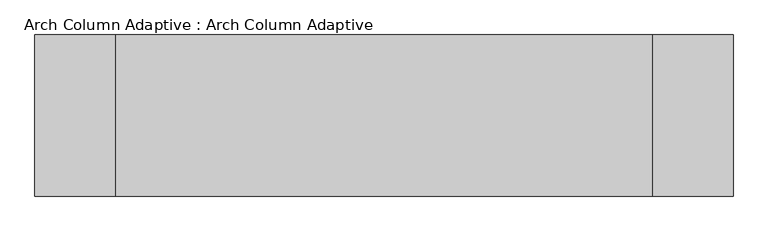
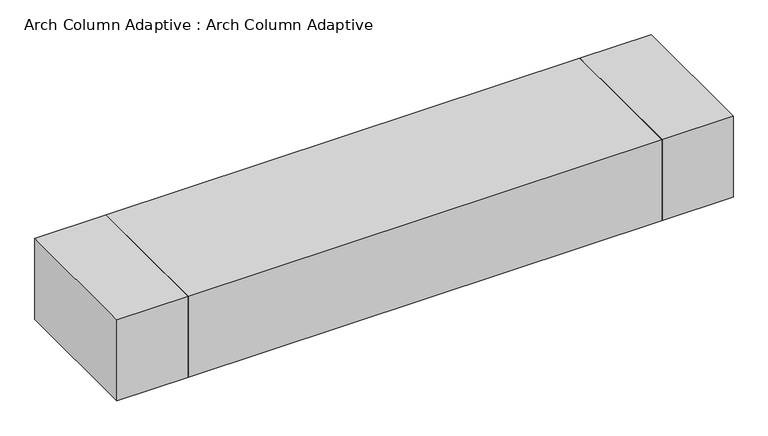
"""IFC4 building model written with IfcOpenShell, lengths in millimetres: proxy geometry, Arch Column Adaptive : Arch Column Adaptive."""

import ifcopenshell
import ifcopenshell.guid

model = None  # the IFC model being written
_history = None  # IfcOwnerHistory: only IFC2X3 demands one
_inside = {}  # id of a spatial element -> (the spatial element, [elements in it])
_under = {}  # id of a project, library or spatial element -> (it, [spatial elements below it])
_declared = {}  # id of a project -> (the project, [libraries it declares])
_typed = {}  # id of a type object -> (the type object, [elements of that type])
_made_of = {}  # id of a material, layer set ... -> (it, [elements and type objects made of it])


def new_model(schema):
    """Start an empty IFC model of exactly this schema.

    Asked for "IFC4X3", IfcOpenShell would pick the latest addendum, in which some entities
    have other attributes; the version numbers below select the first issue.
    IFC2X3 requires an IfcOwnerHistory on every rooted entity: one is made here for all.
    """
    global model, _history
    if schema == "IFC4X3":
        model = ifcopenshell.file(schema_version=(4, 3, 0, 0))
    else:
        model = ifcopenshell.file(schema=schema)
    _inside.clear()
    _under.clear()
    _declared.clear()
    _typed.clear()
    _made_of.clear()
    _history = None
    if model.schema == "IFC2X3":
        org = make("IfcOrganization", Name="unknown")
        user = make(
            "IfcPersonAndOrganization",
            ThePerson=make("IfcPerson", FamilyName="unknown"),
            TheOrganization=org,
        )
        app = make(
            "IfcApplication",
            ApplicationDeveloper=org,
            Version="unknown",
            ApplicationFullName="unknown",
            ApplicationIdentifier="unknown",
        )
        _history = make(
            "IfcOwnerHistory",
            OwningUser=user,
            OwningApplication=app,
            ChangeAction="ADDED",
            CreationDate=0,
        )
    return model


def make(cls, **values):
    """One entity of the class cls with the attributes given. An attribute that is None is left unset."""
    return model.create_entity(
        cls, **{name: value for name, value in values.items() if value is not None}
    )


def rooted(cls, **values):
    """An entity with a GlobalId (a new one), such as an element, a storey or a relation."""
    return make(cls, GlobalId=ifcopenshell.guid.new(), OwnerHistory=_history, **values)


def si_unit(unit_type, name, prefix=None):
    """IfcSIUnit, for example si_unit("LENGTHUNIT", "METRE", prefix="MILLI")."""
    return make("IfcSIUnit", UnitType=unit_type, Prefix=prefix, Name=name)


def assignment(units):
    """IfcUnitAssignment: the units of a project."""
    return None if units is None else make("IfcUnitAssignment", Units=units)


def point(xyz):
    """IfcCartesianPoint."""
    return None if xyz is None else make("IfcCartesianPoint", Coordinates=xyz)


def direction(xyz):
    """IfcDirection."""
    return None if xyz is None else make("IfcDirection", DirectionRatios=xyz)


def frame(location, z_axis=None, x_axis=None):
    """IfcAxis2Placement3D, a coordinate frame: its origin and axes. An axis left out is left unset."""
    return make(
        "IfcAxis2Placement3D",
        Location=point(location),
        Axis=direction(z_axis),
        RefDirection=direction(x_axis),
    )


def origin():
    """The frame at (0, 0, 0) with its axes left unset."""
    return frame((0.0, 0.0, 0.0))


def place(relative_to, where):
    """IfcLocalPlacement: puts the frame where relative to a parent placement (None: the world)."""
    return make(
        "IfcLocalPlacement", PlacementRelTo=relative_to, RelativePlacement=where
    )


def context(
    kind, dimensions, precision=None, world=None, true_north=None, identifier=None
):
    """IfcGeometricRepresentationContext, for example the 3D "Model" context."""
    return make(
        "IfcGeometricRepresentationContext",
        ContextIdentifier=identifier,
        ContextType=kind,
        CoordinateSpaceDimension=dimensions,
        Precision=precision,
        WorldCoordinateSystem=world,
        TrueNorth=true_north,
    )


def project(units=None, contexts=None):
    """IfcProject with its units and contexts."""
    return rooted(
        "IfcProject",
        Name="project",
        RepresentationContexts=contexts,
        UnitsInContext=assignment(units),
    )


def spatial(cls, under=None, at=None, **own):
    """A site, building, storey or space (cls), placed at a placement, below another one or the project."""
    s = rooted(cls, ObjectPlacement=at, **own)
    if under is not None:
        _under.setdefault(under.id(), (under, []))[1].append(s)
    return s


def polyline(points):
    """IfcPolyline through the points."""
    return make("IfcPolyline", Points=[point(p) for p in points])


def outline(outer, holes=None, kind="AREA"):
    """IfcArbitraryClosedProfileDef: a profile drawn as a closed curve; with holes, ...WithVoids."""
    if holes is None:
        return make("IfcArbitraryClosedProfileDef", ProfileType=kind, OuterCurve=outer)
    return make(
        "IfcArbitraryProfileDefWithVoids",
        ProfileType=kind,
        OuterCurve=outer,
        InnerCurves=holes,
    )


def extrude(swept, where, along, depth):
    """IfcExtrudedAreaSolid: the profile swept, set in the frame where, extruded along a direction by depth."""
    return make(
        "IfcExtrudedAreaSolid",
        SweptArea=swept,
        Position=where,
        ExtrudedDirection=direction(along),
        Depth=depth,
    )


def shape(context_of_items, identifier, shape_type, items):
    """IfcShapeRepresentation: the items that make up one representation, for example the "Body"."""
    return make(
        "IfcShapeRepresentation",
        ContextOfItems=context_of_items,
        RepresentationIdentifier=identifier,
        RepresentationType=shape_type,
        Items=items,
    )


def source(mapping_origin, context_of_items, identifier, shape_type, items):
    """IfcRepresentationMap: a shape defined once, which mapped items show again and again."""
    return make(
        "IfcRepresentationMap",
        MappingOrigin=mapping_origin,
        MappedRepresentation=shape(context_of_items, identifier, shape_type, items),
    )


def transform(
    local_origin,
    x_axis=None,
    y_axis=None,
    z_axis=None,
    scale=None,
    scale2=None,
    scale3=None,
    uniform=True,
):
    """IfcCartesianTransformationOperator3D, or its non-uniform kind. x_axis, y_axis, z_axis: its Axis1, 2, 3."""
    if uniform:
        return make(
            "IfcCartesianTransformationOperator3D",
            Axis1=direction(x_axis),
            Axis2=direction(y_axis),
            LocalOrigin=point(local_origin),
            Scale=scale,
            Axis3=direction(z_axis),
        )
    return make(
        "IfcCartesianTransformationOperator3DnonUniform",
        Axis1=direction(x_axis),
        Axis2=direction(y_axis),
        LocalOrigin=point(local_origin),
        Scale=scale,
        Axis3=direction(z_axis),
        Scale2=scale2,
        Scale3=scale3,
    )


def mapped(mapping_source, mapping_target):
    """IfcMappedItem: shows the shape of a source again, moved by a transform."""
    return make(
        "IfcMappedItem", MappingSource=mapping_source, MappingTarget=mapping_target
    )


def made_of(thing, what):
    """Note that an element or type object is made of a material, layer set ...; save() writes the relation."""
    if what is not None:
        _made_of.setdefault(what.id(), (what, []))[1].append(thing)
    return thing


def element(
    cls,
    number,
    at=None,
    inside=None,
    cuts=None,
    type_object=None,
    material=None,
    context=None,
    identifier="Body",
    shape_type=None,
    held_by="IfcProductDefinitionShape",
    body=None,
    shapes=None,
    **own,
):
    """One element of the class cls, such as IfcWall. Its Tag is "e" and its number.

    at: its placement. inside: the storey or other place that contains it. cuts: it is an
    opening in that element (IfcRelVoidsElement). A single representation is given by context,
    identifier, shape_type and body (its items); several are given by shapes. held_by: the class
    of the entity that holds the representations. save() writes the other relations.
    """
    e = rooted(cls, Tag="e%d" % number, ObjectPlacement=at, **own)
    if body is not None:
        shapes = [shape(context, identifier, shape_type, body)]
    if shapes is not None:
        e.Representation = make(held_by, Representations=shapes)
    if inside is not None:
        _inside.setdefault(inside.id(), (inside, []))[1].append(e)
    if cuts is not None:
        rooted(
            "IfcRelVoidsElement", RelatingBuildingElement=cuts, RelatedOpeningElement=e
        )
    if type_object is not None:
        _typed.setdefault(type_object.id(), (type_object, []))[1].append(e)
    return made_of(e, material)


def aggregate(whole, parts):
    """IfcRelAggregates: a whole, such as a stair, and the parts it consists of."""
    return rooted("IfcRelAggregates", RelatingObject=whole, RelatedObjects=parts)


def save(model, path):
    """Write the relations noted so far, then the file.

    IfcRelAggregates (storeys below a building ...), IfcRelContainedInSpatialStructure (elements
    in a storey), IfcRelDefinesByType, IfcRelAssociatesMaterial and IfcRelDeclares: one each for
    every whole, place, type object, material and project.
    """
    for whole, parts in _under.values():
        aggregate(whole, parts)
    for where, things in _inside.values():
        rooted(
            "IfcRelContainedInSpatialStructure",
            RelatedElements=things,
            RelatingStructure=where,
        )
    for kind, things in _typed.values():
        rooted("IfcRelDefinesByType", RelatedObjects=things, RelatingType=kind)
    for what, things in _made_of.values():
        rooted("IfcRelAssociatesMaterial", RelatedObjects=things, RelatingMaterial=what)
    for by, libraries in _declared.values():
        rooted("IfcRelDeclares", RelatingContext=by, RelatedDefinitions=libraries)
    model.write(path)


def arch_column_adaptive_arch_column_adaptive_5d259f20(model_context):
    return source(origin(), model_context, "Body", "SweptSolid", [
        extrude(outline(polyline([(5000.0, -1500.0), (5000.0, 1500.0), (6500.0, 1500.0), (6500.0, -1500.0), (5000.0, -1500.0)])), frame((0.0, 0.0, 46130.0), z_axis=(0.0, 0.0, 1.0), x_axis=(1.0, 0.0, 0.0)), (0.0, 0.0, 1.0), 1800.0),
        extrude(outline(polyline([(-5000.0, 1500.0), (-5000.0, -1500.0), (-6500.0, -1500.0), (-6500.0, 1500.0), (-5000.0, 1500.0)])), frame((0.0, 0.0, 46130.0), z_axis=(0.0, 0.0, 1.0), x_axis=(1.0, 0.0, 0.0)), (0.0, 0.0, 1.0), 1800.0),
        extrude(outline(polyline([(-5000.0, -1500.0), (-5000.0, 1500.0), (5000.0, 1500.0), (5000.0, -1500.0), (-5000.0, -1500.0)])), frame((0.0, 0.0, 46130.0), z_axis=(0.0, 0.0, 1.0), x_axis=(1.0, 0.0, 0.0)), (0.0, 0.0, 1.0), 1800.0),
    ])


if __name__ == "__main__":
    model = new_model("IFC4")
    model_context = context("Model", 3, world=origin())
    ifc_project = project(units=[si_unit("LENGTHUNIT", "METRE", prefix="MILLI")], contexts=[model_context])
    site = spatial("IfcSite", under=ifc_project)
    building = spatial("IfcBuilding", under=site)
    placement = place(None, origin())
    arch_column_adaptive_arch_column_adaptive_shape = arch_column_adaptive_arch_column_adaptive_5d259f20(model_context)
    element("IfcBuildingElementProxy", 1, Name="Arch Column Adaptive : Arch Column Adaptive", ObjectType="Arch Column Adaptive : Arch Column Adaptive", at=placement, inside=building, context=model_context, shape_type="MappedRepresentation", body=[
        mapped(arch_column_adaptive_arch_column_adaptive_shape, transform((0.0, 0.0, 0.0), x_axis=(1.0, 0.0, 0.0), y_axis=(0.0, 1.0, 0.0), z_axis=(0.0, 0.0, 1.0))),
    ])
    save(model, "model.ifc")

# Revit data of these elements
# Type "Arch Column Adaptive : Arch Column Adaptive"
#   Top Width = 3000 mm
#   Length [instance default] = 21000 mm
#   Height [instance default] = 50000 mm
#   Default Elevation = 0
# Element 1 (IfcBuildingElementProxy, "Arch Column Adaptive : Arch Column Adaptive")
#   Height = 46130 mm
